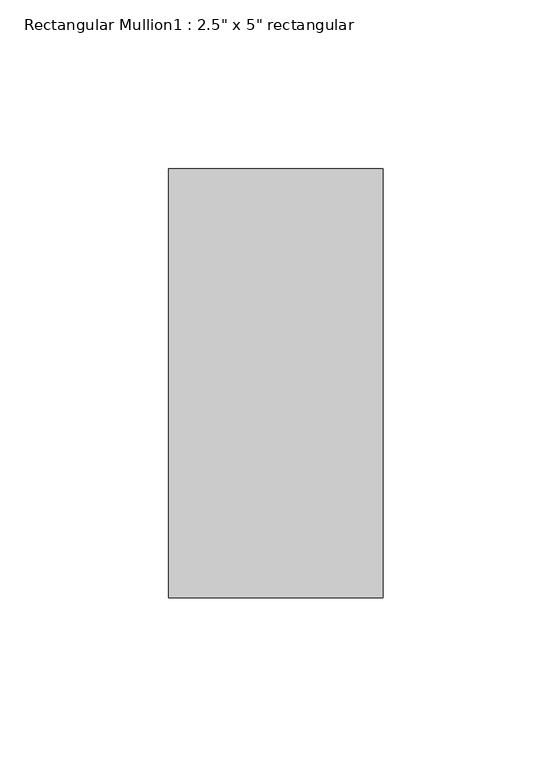
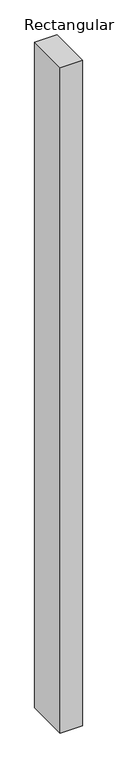
"""IFC4 building model written with IfcOpenShell, lengths in millimetres: member geometry."""

import ifcopenshell
import ifcopenshell.guid

model = None  # the IFC model being written
_history = None  # IfcOwnerHistory: only IFC2X3 demands one
_inside = {}  # id of a spatial element -> (the spatial element, [elements in it])
_under = {}  # id of a project, library or spatial element -> (it, [spatial elements below it])
_declared = {}  # id of a project -> (the project, [libraries it declares])
_typed = {}  # id of a type object -> (the type object, [elements of that type])
_made_of = {}  # id of a material, layer set ... -> (it, [elements and type objects made of it])


def new_model(schema):
    """Start an empty IFC model of exactly this schema.

    Asked for "IFC4X3", IfcOpenShell would pick the latest addendum, in which some entities
    have other attributes; the version numbers below select the first issue.
    IFC2X3 requires an IfcOwnerHistory on every rooted entity: one is made here for all.
    """
    global model, _history
    if schema == "IFC4X3":
        model = ifcopenshell.file(schema_version=(4, 3, 0, 0))
    else:
        model = ifcopenshell.file(schema=schema)
    _inside.clear()
    _under.clear()
    _declared.clear()
    _typed.clear()
    _made_of.clear()
    _history = None
    if model.schema == "IFC2X3":
        org = make("IfcOrganization", Name="unknown")
        user = make(
            "IfcPersonAndOrganization",
            ThePerson=make("IfcPerson", FamilyName="unknown"),
            TheOrganization=org,
        )
        app = make(
            "IfcApplication",
            ApplicationDeveloper=org,
            Version="unknown",
            ApplicationFullName="unknown",
            ApplicationIdentifier="unknown",
        )
        _history = make(
            "IfcOwnerHistory",
            OwningUser=user,
            OwningApplication=app,
            ChangeAction="ADDED",
            CreationDate=0,
        )
    return model


def make(cls, **values):
    """One entity of the class cls with the attributes given. An attribute that is None is left unset."""
    return model.create_entity(
        cls, **{name: value for name, value in values.items() if value is not None}
    )


def rooted(cls, **values):
    """An entity with a GlobalId (a new one), such as an element, a storey or a relation."""
    return make(cls, GlobalId=ifcopenshell.guid.new(), OwnerHistory=_history, **values)


def si_unit(unit_type, name, prefix=None):
    """IfcSIUnit, for example si_unit("LENGTHUNIT", "METRE", prefix="MILLI")."""
    return make("IfcSIUnit", UnitType=unit_type, Prefix=prefix, Name=name)


def assignment(units):
    """IfcUnitAssignment: the units of a project."""
    return None if units is None else make("IfcUnitAssignment", Units=units)


def point(xyz):
    """IfcCartesianPoint."""
    return None if xyz is None else make("IfcCartesianPoint", Coordinates=xyz)


def direction(xyz):
    """IfcDirection."""
    return None if xyz is None else make("IfcDirection", DirectionRatios=xyz)


def frame(location, z_axis=None, x_axis=None):
    """IfcAxis2Placement3D, a coordinate frame: its origin and axes. An axis left out is left unset."""
    return make(
        "IfcAxis2Placement3D",
        Location=point(location),
        Axis=direction(z_axis),
        RefDirection=direction(x_axis),
    )


def origin():
    """The frame at (0, 0, 0) with its axes left unset."""
    return frame((0.0, 0.0, 0.0))


def place(relative_to, where):
    """IfcLocalPlacement: puts the frame where relative to a parent placement (None: the world)."""
    return make(
        "IfcLocalPlacement", PlacementRelTo=relative_to, RelativePlacement=where
    )


def context(
    kind, dimensions, precision=None, world=None, true_north=None, identifier=None
):
    """IfcGeometricRepresentationContext, for example the 3D "Model" context."""
    return make(
        "IfcGeometricRepresentationContext",
        ContextIdentifier=identifier,
        ContextType=kind,
        CoordinateSpaceDimension=dimensions,
        Precision=precision,
        WorldCoordinateSystem=world,
        TrueNorth=true_north,
    )


def project(units=None, contexts=None):
    """IfcProject with its units and contexts."""
    return rooted(
        "IfcProject",
        Name="project",
        RepresentationContexts=contexts,
        UnitsInContext=assignment(units),
    )


def spatial(cls, under=None, at=None, **own):
    """A site, building, storey or space (cls), placed at a placement, below another one or the project."""
    s = rooted(cls, ObjectPlacement=at, **own)
    if under is not None:
        _under.setdefault(under.id(), (under, []))[1].append(s)
    return s


def polyline(points):
    """IfcPolyline through the points."""
    return make("IfcPolyline", Points=[point(p) for p in points])


def outline(outer, holes=None, kind="AREA"):
    """IfcArbitraryClosedProfileDef: a profile drawn as a closed curve; with holes, ...WithVoids."""
    if holes is None:
        return make("IfcArbitraryClosedProfileDef", ProfileType=kind, OuterCurve=outer)
    return make(
        "IfcArbitraryProfileDefWithVoids",
        ProfileType=kind,
        OuterCurve=outer,
        InnerCurves=holes,
    )


def extrude(swept, where, along, depth):
    """IfcExtrudedAreaSolid: the profile swept, set in the frame where, extruded along a direction by depth."""
    return make(
        "IfcExtrudedAreaSolid",
        SweptArea=swept,
        Position=where,
        ExtrudedDirection=direction(along),
        Depth=depth,
    )


def shape(context_of_items, identifier, shape_type, items):
    """IfcShapeRepresentation: the items that make up one representation, for example the "Body"."""
    return make(
        "IfcShapeRepresentation",
        ContextOfItems=context_of_items,
        RepresentationIdentifier=identifier,
        RepresentationType=shape_type,
        Items=items,
    )


def source(mapping_origin, context_of_items, identifier, shape_type, items):
    """IfcRepresentationMap: a shape defined once, which mapped items show again and again."""
    return make(
        "IfcRepresentationMap",
        MappingOrigin=mapping_origin,
        MappedRepresentation=shape(context_of_items, identifier, shape_type, items),
    )


def transform(
    local_origin,
    x_axis=None,
    y_axis=None,
    z_axis=None,
    scale=None,
    scale2=None,
    scale3=None,
    uniform=True,
):
    """IfcCartesianTransformationOperator3D, or its non-uniform kind. x_axis, y_axis, z_axis: its Axis1, 2, 3."""
    if uniform:
        return make(
            "IfcCartesianTransformationOperator3D",
            Axis1=direction(x_axis),
            Axis2=direction(y_axis),
            LocalOrigin=point(local_origin),
            Scale=scale,
            Axis3=direction(z_axis),
        )
    return make(
        "IfcCartesianTransformationOperator3DnonUniform",
        Axis1=direction(x_axis),
        Axis2=direction(y_axis),
        LocalOrigin=point(local_origin),
        Scale=scale,
        Axis3=direction(z_axis),
        Scale2=scale2,
        Scale3=scale3,
    )


def mapped(mapping_source, mapping_target):
    """IfcMappedItem: shows the shape of a source again, moved by a transform."""
    return make(
        "IfcMappedItem", MappingSource=mapping_source, MappingTarget=mapping_target
    )


def made_of(thing, what):
    """Note that an element or type object is made of a material, layer set ...; save() writes the relation."""
    if what is not None:
        _made_of.setdefault(what.id(), (what, []))[1].append(thing)
    return thing


def element(
    cls,
    number,
    at=None,
    inside=None,
    cuts=None,
    type_object=None,
    material=None,
    context=None,
    identifier="Body",
    shape_type=None,
    held_by="IfcProductDefinitionShape",
    body=None,
    shapes=None,
    **own,
):
    """One element of the class cls, such as IfcWall. Its Tag is "e" and its number.

    at: its placement. inside: the storey or other place that contains it. cuts: it is an
    opening in that element (IfcRelVoidsElement). A single representation is given by context,
    identifier, shape_type and body (its items); several are given by shapes. held_by: the class
    of the entity that holds the representations. save() writes the other relations.
    """
    e = rooted(cls, Tag="e%d" % number, ObjectPlacement=at, **own)
    if body is not None:
        shapes = [shape(context, identifier, shape_type, body)]
    if shapes is not None:
        e.Representation = make(held_by, Representations=shapes)
    if inside is not None:
        _inside.setdefault(inside.id(), (inside, []))[1].append(e)
    if cuts is not None:
        rooted(
            "IfcRelVoidsElement", RelatingBuildingElement=cuts, RelatedOpeningElement=e
        )
    if type_object is not None:
        _typed.setdefault(type_object.id(), (type_object, []))[1].append(e)
    return made_of(e, material)


def aggregate(whole, parts):
    """IfcRelAggregates: a whole, such as a stair, and the parts it consists of."""
    return rooted("IfcRelAggregates", RelatingObject=whole, RelatedObjects=parts)


def save(model, path):
    """Write the relations noted so far, then the file.

    IfcRelAggregates (storeys below a building ...), IfcRelContainedInSpatialStructure (elements
    in a storey), IfcRelDefinesByType, IfcRelAssociatesMaterial and IfcRelDeclares: one each for
    every whole, place, type object, material and project.
    """
    for whole, parts in _under.values():
        aggregate(whole, parts)
    for where, things in _inside.values():
        rooted(
            "IfcRelContainedInSpatialStructure",
            RelatedElements=things,
            RelatingStructure=where,
        )
    for kind, things in _typed.values():
        rooted("IfcRelDefinesByType", RelatedObjects=things, RelatingType=kind)
    for what, things in _made_of.values():
        rooted("IfcRelAssociatesMaterial", RelatedObjects=things, RelatingMaterial=what)
    for by, libraries in _declared.values():
        rooted("IfcRelDeclares", RelatingContext=by, RelatedDefinitions=libraries)
    model.write(path)


def member_5e46efc9(model_context):
    return source(origin(), model_context, "Body", "SweptSolid", [
        extrude(outline(polyline([(31.75, 63.5), (31.75, -63.5), (-31.75, -63.5), (-31.75, 63.5), (31.75, 63.5)])), frame((0.0, 0.0, -2021.4166667), z_axis=(0.0, 0.0, 1.0), x_axis=(1.0, 0.0, 0.0)), (0.0, 0.0, 1.0), 2021.4166667),
    ])


if __name__ == "__main__":
    model = new_model("IFC4")
    model_context = context("Model", 3, world=origin())
    ifc_project = project(units=[si_unit("LENGTHUNIT", "METRE", prefix="MILLI")], contexts=[model_context])
    site = spatial("IfcSite", under=ifc_project)
    building = spatial("IfcBuilding", under=site)
    placement = place(None, origin())
    member_shape = member_5e46efc9(model_context)
    element("IfcMember", 1, ObjectType="Rectangular Mullion1 : 2.5\" x 5\" rectangular", at=placement, inside=building, context=model_context, shape_type="MappedRepresentation", body=[
        mapped(member_shape, transform((0.0, 0.0, 0.0), x_axis=(1.0, 0.0, 0.0), y_axis=(0.0, 1.0, 0.0), z_axis=(0.0, 0.0, 1.0))),
    ])
    save(model, "model.ifc")

# Revit data of these elements
# Type "Rectangular Mullion1 : 2.5\" x 5\" rectangular"
#   built-in parameter 1007304 = 0.416667 (stored number, unit not read)
#   built-in parameter 1007301 = 0.104167 (stored number, unit not read)
#   built-in parameter 1007300 = 0.104167 (stored number, unit not read)
# Element 1 (IfcMember, "Rectangular Mullion1 : 2.5\" x 5\" rectangular")
#   Materials on its faces: "support-frame"
# Materials
#   "support-frame": class "Unassigned", colour RGB 233 233 233, transparency 0, Cost = 0
